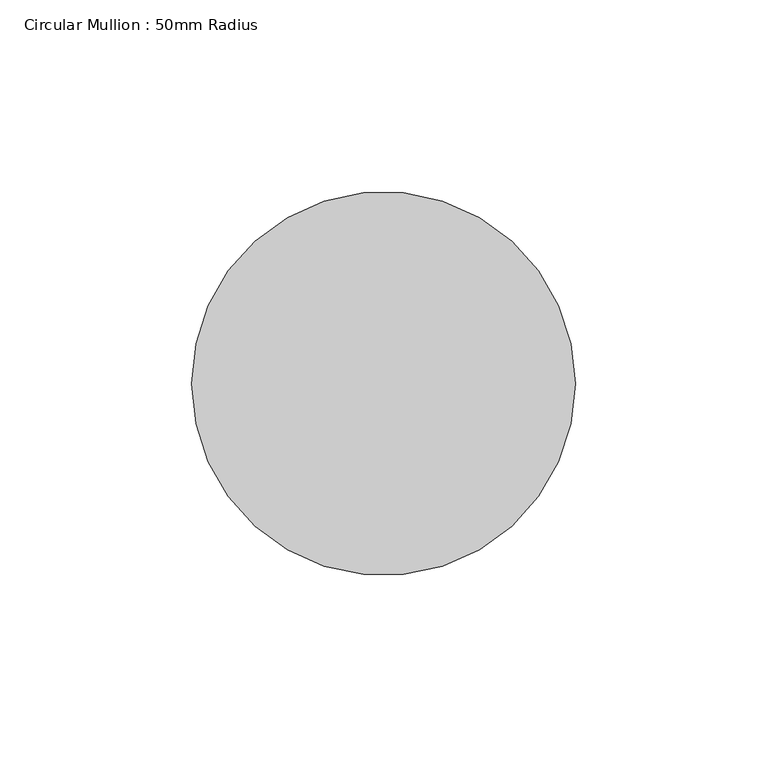
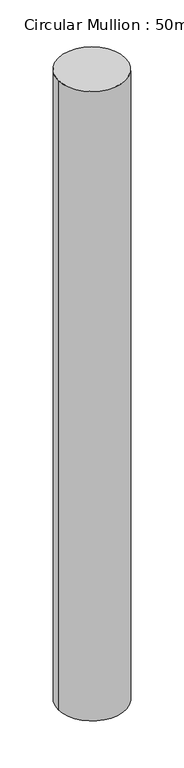
"""IFC4 building model written with IfcOpenShell, lengths in millimetres: member geometry, Circular Mullion : 50mm Radius."""

from ifc_helpers import new_model, si_unit, point, frame, origin, origin_2d, place, context, project, spatial, circle_curve, trimmed, segment, composite_curve, outline, extrude, source, transform, mapped, element, save


def circular_mullion_50mm_radius_4dce5849(model_context):
    return source(origin(), model_context, "Body", "SweptSolid", [
        extrude(outline(composite_curve([segment(trimmed(circle_curve(origin_2d(), 50.0), [point((50.0, 0.0))], [point((-50.0, 0.0))], False, "CARTESIAN"), True, "CONTINUOUS"), segment(trimmed(circle_curve(origin_2d(), 50.0), [point((-50.0, 0.0))], [point((50.0, 0.0))], False, "CARTESIAN"), True, "CONTINUOUS")], self_intersect=False)), frame((0.0, 0.0, -989.9648585), z_axis=(0.0, 0.0, 1.0), x_axis=(1.0, 0.0, 0.0)), (0.0, 0.0, 1.0), 989.9648585),
    ])


if __name__ == "__main__":
    model = new_model("IFC4")
    model_context = context("Model", 3, world=origin())
    ifc_project = project(units=[si_unit("LENGTHUNIT", "METRE", prefix="MILLI")], contexts=[model_context])
    site = spatial("IfcSite", under=ifc_project)
    building = spatial("IfcBuilding", under=site)
    placement = place(None, origin())
    circular_mullion_50mm_radius_shape = circular_mullion_50mm_radius_4dce5849(model_context)
    element("IfcMember", 1, ObjectType="Circular Mullion : 50mm Radius", at=placement, inside=building, context=model_context, shape_type="MappedRepresentation", body=[
        mapped(circular_mullion_50mm_radius_shape, transform((0.0, 0.0, 0.0), x_axis=(1.0, 0.0, 0.0), y_axis=(0.0, 1.0, 0.0), z_axis=(0.0, 0.0, 1.0))),
    ])
    save(model, "model.ifc")

# Revit data of these elements
# Type "Circular Mullion : 50mm Radius"
#   built-in parameter 1007350 = 0.164042 (stored number, unit not read)
# Element 1 (IfcMember, "Circular Mullion : 50mm Radius")
#   Materials on its faces: "Aluminium"
# Materials
#   "Aluminium": class "Metal", colour RGB 247 247 247, transparency 0, Description = "Aluminium 6061", Cost = 0
